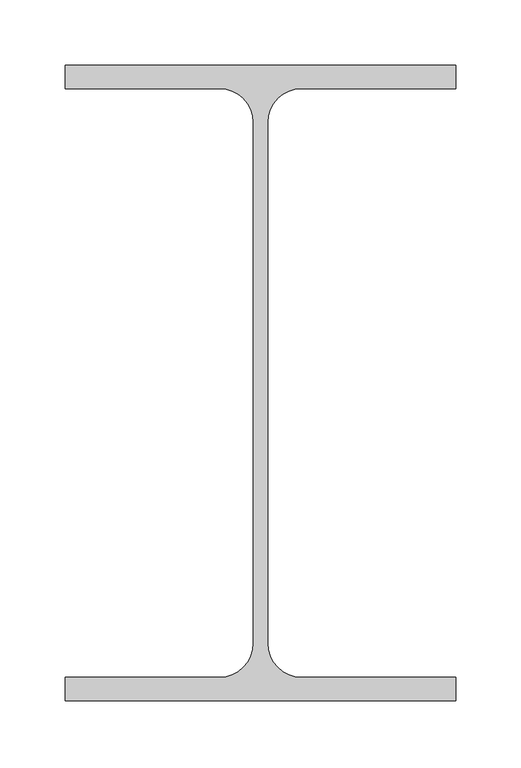
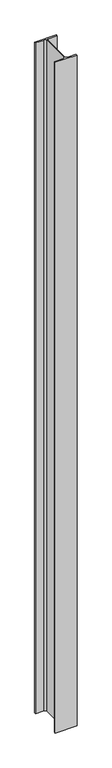
"""IFC4 building model written with IfcOpenShell, lengths in millimetres: column geometry, 0912_Steel Column_H_KSD3502 : H_SC_ASC_H-488x300x11x18."""

import ifcopenshell
import ifcopenshell.guid

model = None  # the IFC model being written
_history = None  # IfcOwnerHistory: only IFC2X3 demands one
_inside = {}  # id of a spatial element -> (the spatial element, [elements in it])
_under = {}  # id of a project, library or spatial element -> (it, [spatial elements below it])
_declared = {}  # id of a project -> (the project, [libraries it declares])
_typed = {}  # id of a type object -> (the type object, [elements of that type])
_made_of = {}  # id of a material, layer set ... -> (it, [elements and type objects made of it])


def new_model(schema):
    """Start an empty IFC model of exactly this schema.

    Asked for "IFC4X3", IfcOpenShell would pick the latest addendum, in which some entities
    have other attributes; the version numbers below select the first issue.
    IFC2X3 requires an IfcOwnerHistory on every rooted entity: one is made here for all.
    """
    global model, _history
    if schema == "IFC4X3":
        model = ifcopenshell.file(schema_version=(4, 3, 0, 0))
    else:
        model = ifcopenshell.file(schema=schema)
    _inside.clear()
    _under.clear()
    _declared.clear()
    _typed.clear()
    _made_of.clear()
    _history = None
    if model.schema == "IFC2X3":
        org = make("IfcOrganization", Name="unknown")
        user = make(
            "IfcPersonAndOrganization",
            ThePerson=make("IfcPerson", FamilyName="unknown"),
            TheOrganization=org,
        )
        app = make(
            "IfcApplication",
            ApplicationDeveloper=org,
            Version="unknown",
            ApplicationFullName="unknown",
            ApplicationIdentifier="unknown",
        )
        _history = make(
            "IfcOwnerHistory",
            OwningUser=user,
            OwningApplication=app,
            ChangeAction="ADDED",
            CreationDate=0,
        )
    return model


def make(cls, **values):
    """One entity of the class cls with the attributes given. An attribute that is None is left unset."""
    return model.create_entity(
        cls, **{name: value for name, value in values.items() if value is not None}
    )


def rooted(cls, **values):
    """An entity with a GlobalId (a new one), such as an element, a storey or a relation."""
    return make(cls, GlobalId=ifcopenshell.guid.new(), OwnerHistory=_history, **values)


def si_unit(unit_type, name, prefix=None):
    """IfcSIUnit, for example si_unit("LENGTHUNIT", "METRE", prefix="MILLI")."""
    return make("IfcSIUnit", UnitType=unit_type, Prefix=prefix, Name=name)


def assignment(units):
    """IfcUnitAssignment: the units of a project."""
    return None if units is None else make("IfcUnitAssignment", Units=units)


def point(xyz):
    """IfcCartesianPoint."""
    return None if xyz is None else make("IfcCartesianPoint", Coordinates=xyz)


def direction(xyz):
    """IfcDirection."""
    return None if xyz is None else make("IfcDirection", DirectionRatios=xyz)


def frame(location, z_axis=None, x_axis=None):
    """IfcAxis2Placement3D, a coordinate frame: its origin and axes. An axis left out is left unset."""
    return make(
        "IfcAxis2Placement3D",
        Location=point(location),
        Axis=direction(z_axis),
        RefDirection=direction(x_axis),
    )


def frame_2d(location, x_axis=None):
    """IfcAxis2Placement2D, a coordinate frame in the plane: its origin and x axis."""
    return make(
        "IfcAxis2Placement2D", Location=point(location), RefDirection=direction(x_axis)
    )


def origin():
    """The frame at (0, 0, 0) with its axes left unset."""
    return frame((0.0, 0.0, 0.0))


def place(relative_to, where):
    """IfcLocalPlacement: puts the frame where relative to a parent placement (None: the world)."""
    return make(
        "IfcLocalPlacement", PlacementRelTo=relative_to, RelativePlacement=where
    )


def context(
    kind, dimensions, precision=None, world=None, true_north=None, identifier=None
):
    """IfcGeometricRepresentationContext, for example the 3D "Model" context."""
    return make(
        "IfcGeometricRepresentationContext",
        ContextIdentifier=identifier,
        ContextType=kind,
        CoordinateSpaceDimension=dimensions,
        Precision=precision,
        WorldCoordinateSystem=world,
        TrueNorth=true_north,
    )


def project(units=None, contexts=None):
    """IfcProject with its units and contexts."""
    return rooted(
        "IfcProject",
        Name="project",
        RepresentationContexts=contexts,
        UnitsInContext=assignment(units),
    )


def spatial(cls, under=None, at=None, **own):
    """A site, building, storey or space (cls), placed at a placement, below another one or the project."""
    s = rooted(cls, ObjectPlacement=at, **own)
    if under is not None:
        _under.setdefault(under.id(), (under, []))[1].append(s)
    return s


def polyline(points):
    """IfcPolyline through the points."""
    return make("IfcPolyline", Points=[point(p) for p in points])


def circle_curve(where, radius):
    """IfcCircle in the frame where."""
    return make("IfcCircle", Position=where, Radius=radius)


def trimmed(basis, trim1, trim2, sense, master):
    """IfcTrimmedCurve: the piece of a basis curve between two trims."""
    return make(
        "IfcTrimmedCurve",
        BasisCurve=basis,
        Trim1=trim1,
        Trim2=trim2,
        SenseAgreement=sense,
        MasterRepresentation=master,
    )


def segment(curve, same_sense, transition):
    """IfcCompositeCurveSegment."""
    return make(
        "IfcCompositeCurveSegment",
        Transition=transition,
        SameSense=same_sense,
        ParentCurve=curve,
    )


def composite_curve(segments, self_intersect=None):
    """IfcCompositeCurve: segments joined end to end."""
    return make("IfcCompositeCurve", Segments=segments, SelfIntersect=self_intersect)


def outline(outer, holes=None, kind="AREA"):
    """IfcArbitraryClosedProfileDef: a profile drawn as a closed curve; with holes, ...WithVoids."""
    if holes is None:
        return make("IfcArbitraryClosedProfileDef", ProfileType=kind, OuterCurve=outer)
    return make(
        "IfcArbitraryProfileDefWithVoids",
        ProfileType=kind,
        OuterCurve=outer,
        InnerCurves=holes,
    )


def extrude(swept, where, along, depth):
    """IfcExtrudedAreaSolid: the profile swept, set in the frame where, extruded along a direction by depth."""
    return make(
        "IfcExtrudedAreaSolid",
        SweptArea=swept,
        Position=where,
        ExtrudedDirection=direction(along),
        Depth=depth,
    )


def shape(context_of_items, identifier, shape_type, items):
    """IfcShapeRepresentation: the items that make up one representation, for example the "Body"."""
    return make(
        "IfcShapeRepresentation",
        ContextOfItems=context_of_items,
        RepresentationIdentifier=identifier,
        RepresentationType=shape_type,
        Items=items,
    )


def source(mapping_origin, context_of_items, identifier, shape_type, items):
    """IfcRepresentationMap: a shape defined once, which mapped items show again and again."""
    return make(
        "IfcRepresentationMap",
        MappingOrigin=mapping_origin,
        MappedRepresentation=shape(context_of_items, identifier, shape_type, items),
    )


def transform(
    local_origin,
    x_axis=None,
    y_axis=None,
    z_axis=None,
    scale=None,
    scale2=None,
    scale3=None,
    uniform=True,
):
    """IfcCartesianTransformationOperator3D, or its non-uniform kind. x_axis, y_axis, z_axis: its Axis1, 2, 3."""
    if uniform:
        return make(
            "IfcCartesianTransformationOperator3D",
            Axis1=direction(x_axis),
            Axis2=direction(y_axis),
            LocalOrigin=point(local_origin),
            Scale=scale,
            Axis3=direction(z_axis),
        )
    return make(
        "IfcCartesianTransformationOperator3DnonUniform",
        Axis1=direction(x_axis),
        Axis2=direction(y_axis),
        LocalOrigin=point(local_origin),
        Scale=scale,
        Axis3=direction(z_axis),
        Scale2=scale2,
        Scale3=scale3,
    )


def mapped(mapping_source, mapping_target):
    """IfcMappedItem: shows the shape of a source again, moved by a transform."""
    return make(
        "IfcMappedItem", MappingSource=mapping_source, MappingTarget=mapping_target
    )


def made_of(thing, what):
    """Note that an element or type object is made of a material, layer set ...; save() writes the relation."""
    if what is not None:
        _made_of.setdefault(what.id(), (what, []))[1].append(thing)
    return thing


def element(
    cls,
    number,
    at=None,
    inside=None,
    cuts=None,
    type_object=None,
    material=None,
    context=None,
    identifier="Body",
    shape_type=None,
    held_by="IfcProductDefinitionShape",
    body=None,
    shapes=None,
    **own,
):
    """One element of the class cls, such as IfcWall. Its Tag is "e" and its number.

    at: its placement. inside: the storey or other place that contains it. cuts: it is an
    opening in that element (IfcRelVoidsElement). A single representation is given by context,
    identifier, shape_type and body (its items); several are given by shapes. held_by: the class
    of the entity that holds the representations. save() writes the other relations.
    """
    e = rooted(cls, Tag="e%d" % number, ObjectPlacement=at, **own)
    if body is not None:
        shapes = [shape(context, identifier, shape_type, body)]
    if shapes is not None:
        e.Representation = make(held_by, Representations=shapes)
    if inside is not None:
        _inside.setdefault(inside.id(), (inside, []))[1].append(e)
    if cuts is not None:
        rooted(
            "IfcRelVoidsElement", RelatingBuildingElement=cuts, RelatedOpeningElement=e
        )
    if type_object is not None:
        _typed.setdefault(type_object.id(), (type_object, []))[1].append(e)
    return made_of(e, material)


def aggregate(whole, parts):
    """IfcRelAggregates: a whole, such as a stair, and the parts it consists of."""
    return rooted("IfcRelAggregates", RelatingObject=whole, RelatedObjects=parts)


def save(model, path):
    """Write the relations noted so far, then the file.

    IfcRelAggregates (storeys below a building ...), IfcRelContainedInSpatialStructure (elements
    in a storey), IfcRelDefinesByType, IfcRelAssociatesMaterial and IfcRelDeclares: one each for
    every whole, place, type object, material and project.
    """
    for whole, parts in _under.values():
        aggregate(whole, parts)
    for where, things in _inside.values():
        rooted(
            "IfcRelContainedInSpatialStructure",
            RelatedElements=things,
            RelatingStructure=where,
        )
    for kind, things in _typed.values():
        rooted("IfcRelDefinesByType", RelatedObjects=things, RelatingType=kind)
    for what, things in _made_of.values():
        rooted("IfcRelAssociatesMaterial", RelatedObjects=things, RelatingMaterial=what)
    for by, libraries in _declared.values():
        rooted("IfcRelDeclares", RelatingContext=by, RelatedDefinitions=libraries)
    model.write(path)


def column_bd22218f(model_context):
    return source(origin(), model_context, "Body", "SweptSolid", [
        extrude(outline(composite_curve([segment(polyline([(150.0, 244.0), (150.0, 226.0), (31.5, 226.0)]), True, "CONTINUOUS"), segment(trimmed(circle_curve(frame_2d((31.5, 200.0)), 26.0), [point((31.5, 226.0))], [point((5.5, 200.0))], True, "CARTESIAN"), True, "CONTINUOUS"), segment(polyline([(5.5, 200.0), (5.5, -200.0)]), True, "CONTINUOUS"), segment(trimmed(circle_curve(frame_2d((31.5, -200.0)), 26.0), [point((5.5, -200.0))], [point((31.5, -226.0))], True, "CARTESIAN"), True, "CONTINUOUS"), segment(polyline([(31.5, -226.0), (150.0, -226.0), (150.0, -244.0), (-150.0, -244.0), (-150.0, -226.0), (-31.5, -226.0)]), True, "CONTINUOUS"), segment(trimmed(circle_curve(frame_2d((-31.5, -200.0)), 26.0), [point((-31.5, -226.0))], [point((-5.5, -200.0))], True, "CARTESIAN"), True, "CONTINUOUS"), segment(polyline([(-5.5, -200.0), (-5.5, 200.0)]), True, "CONTINUOUS"), segment(trimmed(circle_curve(frame_2d((-31.5, 200.0)), 26.0), [point((-5.5, 200.0))], [point((-31.5, 226.0))], True, "CARTESIAN"), True, "CONTINUOUS"), segment(polyline([(-31.5, 226.0), (-150.0, 226.0), (-150.0, 244.0), (150.0, 244.0)]), True, "CONTINUOUS")], self_intersect=False)), frame((0.0, 0.0, 7538.9720055), z_axis=(0.0, 0.0, 1.0), x_axis=(1.0, 0.0, 0.0)), (0.0, 0.0, 1.0), 9761.0),
    ])


if __name__ == "__main__":
    model = new_model("IFC4")
    model_context = context("Model", 3, world=origin())
    ifc_project = project(units=[si_unit("LENGTHUNIT", "METRE", prefix="MILLI")], contexts=[model_context])
    site = spatial("IfcSite", under=ifc_project)
    building = spatial("IfcBuilding", under=site)
    placement = place(None, origin())
    column_shape = column_bd22218f(model_context)
    element("IfcColumn", 1, ObjectType="0912_Steel Column_H_KSD3502 : H_SC_ASC_H-488x300x11x18", at=placement, inside=building, context=model_context, shape_type="MappedRepresentation", body=[
        mapped(column_shape, transform((0.0, 0.0, 0.0), x_axis=(1.0, 0.0, 0.0), y_axis=(0.0, 1.0, 0.0), z_axis=(0.0, 0.0, 1.0))),
    ])
    save(model, "model.ifc")

# Revit data of these elements
# Type "0912_Steel Column_H_KSD3502 : H_SC_ASC_H-488x300x11x18"
#   H_WM Code_1 = "S01AA002-00001 | Main Steel Structure Fabrication Work | Shelter/Building | Medium Steel - Standard (90KG/M>Weight≥30KG/M) | Material: (   )"
#   H_WM Code_2 = "S03AA028-00001 | Main Steel Structure Erection Work | Shelter/Building | Medium Steel (90KG/M>Weight≥30KG/M) | Material: (   )"
#   H_WM Code_3 = "S01AA010-00001 | Main Steel Structure Fabrication Work | Shelter/Building | Steel Painting/Coating | for Non-Fireproofed Steel Surface, Surface Preparation, Primer, Second & Final Coat | Material: (   )"
#   H_Q'ty Cal Type Tag = "SC-Q2"
#   Width = 30.0 cm
#   Web Thickness = 1.1 cm
#   Web Fillet = 2.6 cm
#   Warping Constant = 4473230.0 cm⁶
#   Torsional Moment of Inertia = 137.492 cm⁴
#   Section Area = 163.5 cm²
#   Plastic Modulus weak axis = 830.0 cm³
#   Plastic Modulus strong axis = 3230.0 cm³
#   Perimeter = 2.11 m²/m
#   Nominal Weight = 128.00 kgf/m
#   Moment of Inertia weak axis = 8110.00 cm⁴
#   Moment of Inertia strong axis = 71000.00 cm⁴
#   Height = 48.8 cm
#   Flange Thickness = 1.8 cm
#   Elastic Modulus weak axis = 541.0 cm³
#   Elastic Modulus strong axis = 2910.0 cm³
#   Centroid Vertical = 24.4 cm
#   Centroid Horizontal = 15.0 cm
#   Structural Material [instance default] = Steel, 45-345
#   Section Name Key = ""
#   Bolt Spacing = 0
#   Assembly Code = ""
# Element 1 (IfcColumn, "0912_Steel Column_H_KSD3502 : H_SC_ASC_H-488x300x11x18")
#   Structural Material = none
# Materials
#   "Steel, 45-345": class "Metal", colour RGB 189 187 185, transparency 0, Description = "Steel 345 MPa", Cost = 0
